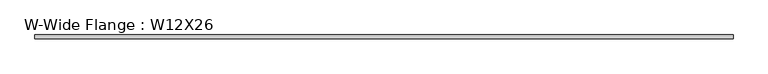
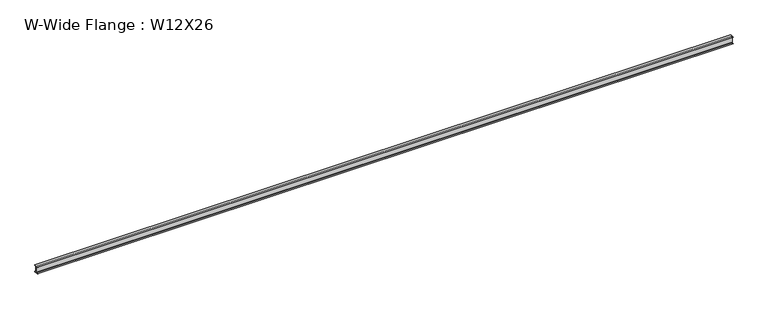
"""IFC4 building model written with IfcOpenShell, lengths in millimetres: beam geometry, W-Wide Flange : W12X26."""

from ifc_helpers import new_model, si_unit, point, frame, frame_2d, origin, place, context, project, spatial, polyline, circle_curve, trimmed, segment, composite_curve, outline, extrude, source, transform, mapped, element, save


def w_wide_flange_w12x26_6694fb91(model_context):
    return source(origin(), model_context, "Body", "SweptSolid", [
        extrude(outline(composite_curve([segment(polyline([(82.4011719, -145.5539063), (82.4011719, -155.178125), (-82.4011719, -155.178125), (-82.4011719, -145.5539063), (-20.2902344, -145.5539063)]), True, "CONTINUOUS"), segment(trimmed(circle_curve(frame_2d((-20.2902344, -128.190625)), 17.3632812), [point((-20.2902344, -145.5539063))], [point((-2.9269531, -128.190625))], True, "CARTESIAN"), True, "CONTINUOUS"), segment(polyline([(-2.9269531, -128.190625), (-2.9269531, 128.190625)]), True, "CONTINUOUS"), segment(trimmed(circle_curve(frame_2d((-20.2902344, 128.190625)), 17.3632812), [point((-2.9269531, 128.190625))], [point((-20.2902344, 145.5539062))], True, "CARTESIAN"), True, "CONTINUOUS"), segment(polyline([(-20.2902344, 145.5539062), (-82.4011719, 145.5539062), (-82.4011719, 155.178125), (82.4011719, 155.178125), (82.4011719, 145.5539062), (20.2902344, 145.5539062)]), True, "CONTINUOUS"), segment(trimmed(circle_curve(frame_2d((20.2902344, 128.190625)), 17.3632812), [point((20.2902344, 145.5539062))], [point((2.9269531, 128.190625))], True, "CARTESIAN"), True, "CONTINUOUS"), segment(polyline([(2.9269531, 128.190625), (2.9269531, -128.190625)]), True, "CONTINUOUS"), segment(trimmed(circle_curve(frame_2d((20.2902344, -128.190625)), 17.3632812), [point((2.9269531, -128.190625))], [point((20.2902344, -145.5539063))], True, "CARTESIAN"), True, "CONTINUOUS"), segment(polyline([(20.2902344, -145.5539063), (82.4011719, -145.5539063)]), True, "CONTINUOUS")], self_intersect=False)), frame((-15054.2625, 0.0, 0.0), z_axis=(1.0, 0.0, 0.0), x_axis=(0.0, 1.0, 0.0)), (0.0, 0.0, 1.0), 30218.0625),
    ])


if __name__ == "__main__":
    model = new_model("IFC4")
    model_context = context("Model", 3, world=origin())
    ifc_project = project(units=[si_unit("LENGTHUNIT", "METRE", prefix="MILLI")], contexts=[model_context])
    site = spatial("IfcSite", under=ifc_project)
    building = spatial("IfcBuilding", under=site)
    placement = place(None, origin())
    w_wide_flange_w12x26_shape = w_wide_flange_w12x26_6694fb91(model_context)
    element("IfcBeam", 1, ObjectType="W-Wide Flange : W12X26", at=placement, inside=building, context=model_context, shape_type="MappedRepresentation", body=[
        mapped(w_wide_flange_w12x26_shape, transform((0.0, 0.0, 0.0), x_axis=(1.0, 0.0, 0.0), y_axis=(0.0, 1.0, 0.0), z_axis=(0.0, 0.0, 1.0))),
    ])
    save(model, "model.ifc")

# Revit data of these elements
# Type "W-Wide Flange : W12X26"
#   Assembly Code = "B10"
#   W = 26
#   Length [instance default] = 5' - 0"
#   bf = 0' - 6 125/256"
#   d = 1' - 0 7/32"
#   k = 0' - 1 1/16"
#   k2 = 0' - 0 175/256"
#   tf = 0' - 0 97/256"
#   tw = 0' - 0 59/256"
#   A = 0.053125 SF
#   Structural Material [instance default] = none
